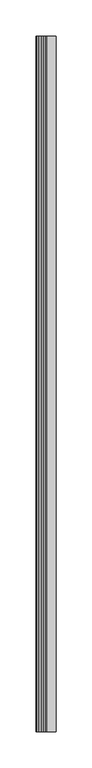
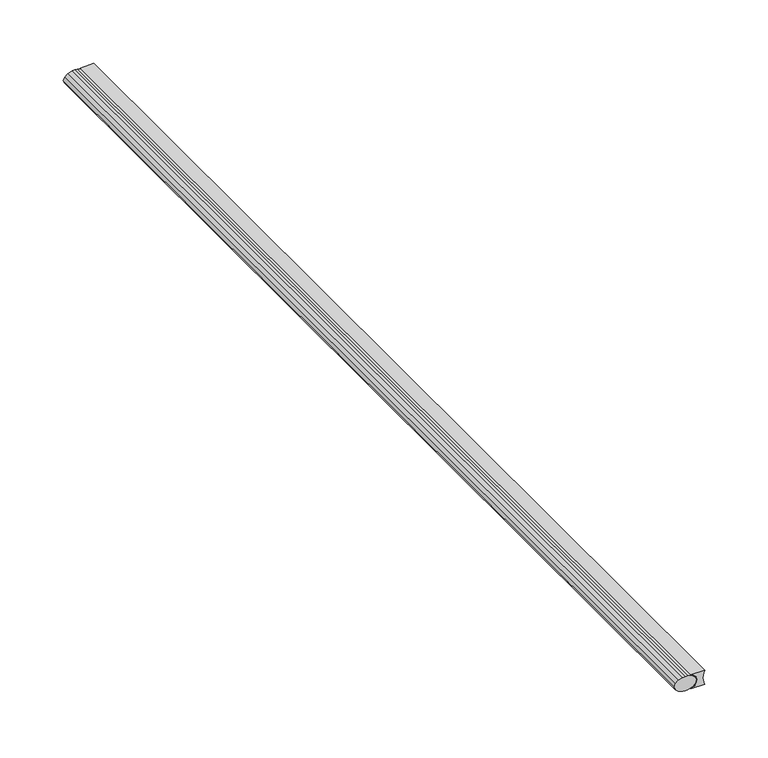
"""IFC4 building model written with IfcOpenShell, lengths in millimetres: proxy geometry, Generic Models 7:Generic Models 1:1:Generic Models 1:1 : Generic Models 7:Generic Models 1:337419:53 : Generic Models 7:Generic Models 1:1:Generic Models 1:1 : Generic Models 7:Generic Models 1:337419:306201."""

from ifc_helpers import new_model, si_unit, frame, origin, place, context, project, spatial, polyline, outline, extrude, source, transform, mapped, element, save


def generic_models_301acde3(model_context):
    return source(origin(), model_context, "Body", "SweptSolid", [
        extrude(outline(polyline([(3715.5279199, 560350.0316569), (3714.7079581, 560351.8576094), (3712.4082526, 560354.6371919), (3709.5423421, 560355.9114465), (3706.5585721, 560355.4810277), (3703.9237255, 560353.4132707), (3702.05, 560350.0316569), (3702.05, 560362.4867239), (3704.0998393, 560361.6856715), (3708.7889599, 560361.0198706), (3713.4780806, 560361.6856715), (3715.5279199, 560362.4867239), (3715.5279199, 560350.0316569)])), frame((0.0, -546590.0795795, 0.0), z_axis=(0.0, 1.0, 0.0), x_axis=(0.0, 0.0, 1.0)), (0.0, 0.0, 1.0), 961.8131955),
        extrude(outline(polyline([(3715.3589601, 560342.7655012), (3714.057691, 560338.7123315), (3711.7128851, 560335.9074511), (3708.7889599, 560334.9064008), (3705.8650348, 560335.9074511), (3703.5202289, 560338.7123315), (3702.2189598, 560342.7655012), (3702.05, 560345.0148407), (3702.2189598, 560347.2641802), (3703.5202289, 560351.3173499), (3705.8650348, 560354.1222304), (3708.7889599, 560355.1232806), (3711.7128851, 560354.1222304), (3714.057691, 560351.3173499), (3715.3589601, 560347.2641802), (3715.5279199, 560345.0148407), (3715.3589601, 560342.7655012)])), frame((0.0, -546590.0795795, 0.0), z_axis=(0.0, 1.0, 0.0), x_axis=(0.0, 0.0, 1.0)), (0.0, 0.0, 1.0), 961.8131955),
    ])


if __name__ == "__main__":
    model = new_model("IFC4")
    model_context = context("Model", 3, world=origin())
    ifc_project = project(units=[si_unit("LENGTHUNIT", "METRE", prefix="MILLI")], contexts=[model_context])
    site = spatial("IfcSite", under=ifc_project)
    building = spatial("IfcBuilding", under=site)
    placement = place(None, origin())
    generic_models_shape = generic_models_301acde3(model_context)
    element("IfcBuildingElementProxy", 1, Name="Generic Models 7:Generic Models 1:1:Generic Models 1:1 : Generic Models 7:Generic Models 1:337419:53 : Generic Models 7:Generic Models 1:1:Generic Models 1:1 : Generic Models 7:Generic Models 1:337419:306201", ObjectType="Generic Models 7:Generic Models 1:1:Generic Models 1:1 : Generic Models 7:Generic Models 1:337419:53 : Generic Models 7:Generic Models 1:1:Generic Models 1:1 : Generic Models 7:Generic Models 1:337419:306201", at=placement, inside=building, context=model_context, shape_type="MappedRepresentation", body=[
        mapped(generic_models_shape, transform((0.0, 0.0, 0.0), x_axis=(1.0, 0.0, 0.0), y_axis=(0.0, 1.0, 0.0), z_axis=(0.0, 0.0, 1.0))),
    ])
    save(model, "model.ifc")

# Revit data of these elements
# Type "Generic Models 7:Generic Models 1:1:Generic Models 1:1 : Generic Models 7:Generic Models 1:337419:53 : Generic Models 7:Generic Models 1:1:Generic Models 1:1 : Generic Models 7:Generic Models 1:337419:306201"
#   NameOverride = "Generic Models 7:Generic Models 1:1:Generic Models 1:1 : Generic Models 7:Generic Models 1:337419:306201"
#   ObjectTypeOverride = "Generic Models 1:1 : Generic Models 7:Generic Models 1:337419"
#   Reference = "Generic Models 1"
#   Tag = "306201"
# Element 1 (IfcBuildingElementProxy, "Generic Models 7:Generic Models 1:1:Generic Models 1:1 : Generic Models 7:Generic Models 1:337419:53 : Generic Models 7:Generic Models 1:1:Generic Models 1:1 : Generic Models 7:Generic Models 1:337419:306201")
#   Materials on its faces: "SEMI-RIGID EPOXY SEALANT W/ BACKROD (REMOVE TEMP. JOINT FORM)"
# Materials
#   "SEMI-RIGID EPOXY SEALANT W/ BACKROD (REMOVE TEMP. JOINT FORM)": class "Unassigned", colour RGB 120 120 120, transparency 0, Cost = 0
